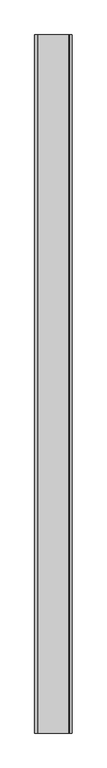
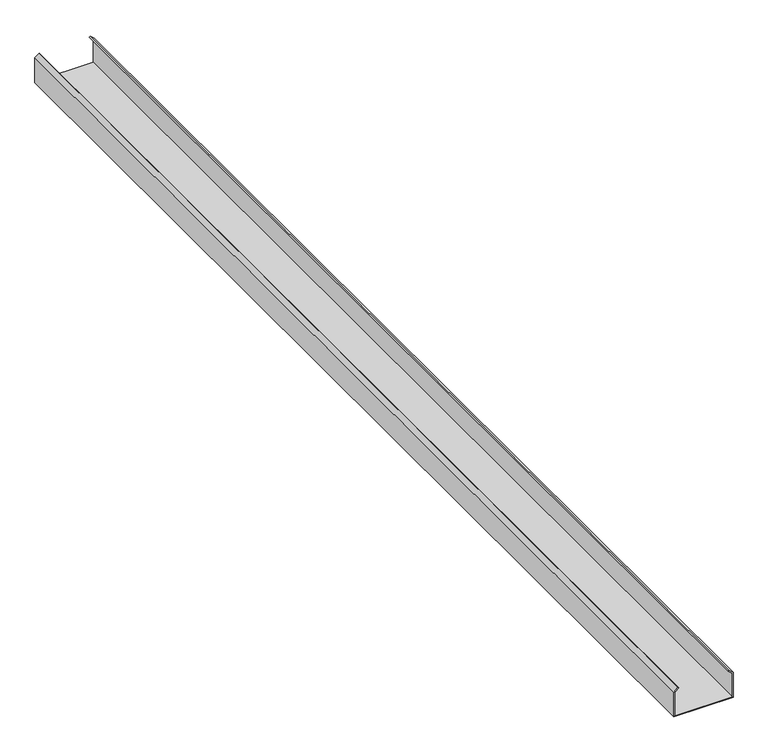
"""IFC4 building model written with IfcOpenShell, lengths in millimetres: proxy geometry, Generic Models 7:Generic Models 1:1:Generic Models 1:1 : Generic Models 7:Generic Models 1:337419:51 : Generic Models 7:Generic Models 1:1:Generic Models 1:1 : Generic Models 7:Generic Models 1:337419:306201."""

from ifc_helpers import new_model, si_unit, frame, origin, place, context, project, spatial, polyline, outline, extrude, source, transform, mapped, element, save


def generic_models_450da2eb(model_context):
    return source(origin(), model_context, "Body", "SweptSolid", [
        extrude(outline(polyline([(3617.9125, 560568.8617239), (3706.8125, 560568.8617239), (3719.057604, 560554.2685773), (3716.9294367, 560552.482833), (3705.517039, 560566.0835989), (3620.690625, 560566.0835989), (3620.690625, 560368.4398489), (3705.517039, 560368.4398489), (3716.9294367, 560382.0406149), (3719.057604, 560380.2548706), (3706.8125, 560365.6617239), (3617.9125, 560365.6617239), (3617.9125, 560568.8617239)])), frame((0.0, -546971.2913841, 0.0), z_axis=(0.0, 1.0, 0.0), x_axis=(0.0, 0.0, 1.0)), (0.0, 0.0, 1.0), 3787.775),
    ])


if __name__ == "__main__":
    model = new_model("IFC4")
    model_context = context("Model", 3, world=origin())
    ifc_project = project(units=[si_unit("LENGTHUNIT", "METRE", prefix="MILLI")], contexts=[model_context])
    site = spatial("IfcSite", under=ifc_project)
    building = spatial("IfcBuilding", under=site)
    placement = place(None, origin())
    generic_models_shape = generic_models_450da2eb(model_context)
    element("IfcBuildingElementProxy", 1, Name="Generic Models 7:Generic Models 1:1:Generic Models 1:1 : Generic Models 7:Generic Models 1:337419:51 : Generic Models 7:Generic Models 1:1:Generic Models 1:1 : Generic Models 7:Generic Models 1:337419:306201", ObjectType="Generic Models 7:Generic Models 1:1:Generic Models 1:1 : Generic Models 7:Generic Models 1:337419:51 : Generic Models 7:Generic Models 1:1:Generic Models 1:1 : Generic Models 7:Generic Models 1:337419:306201", at=placement, inside=building, context=model_context, shape_type="MappedRepresentation", body=[
        mapped(generic_models_shape, transform((0.0, 0.0, 0.0), x_axis=(1.0, 0.0, 0.0), y_axis=(0.0, 1.0, 0.0), z_axis=(0.0, 0.0, 1.0))),
    ])
    save(model, "model.ifc")

# Revit data of these elements
# Type "Generic Models 7:Generic Models 1:1:Generic Models 1:1 : Generic Models 7:Generic Models 1:337419:51 : Generic Models 7:Generic Models 1:1:Generic Models 1:1 : Generic Models 7:Generic Models 1:337419:306201"
#   NameOverride = "Generic Models 7:Generic Models 1:1:Generic Models 1:1 : Generic Models 7:Generic Models 1:337419:306201"
#   ObjectTypeOverride = "Generic Models 1:1 : Generic Models 7:Generic Models 1:337419"
#   Reference = "Generic Models 1"
#   Tag = "306201"
# Element 1 (IfcBuildingElementProxy, "Generic Models 7:Generic Models 1:1:Generic Models 1:1 : Generic Models 7:Generic Models 1:337419:51 : Generic Models 7:Generic Models 1:1:Generic Models 1:1 : Generic Models 7:Generic Models 1:337419:306201")
#   Materials on its faces: "CEE' SECTION (8.0x3.5C - SEE STRUCT. DWGS)"
# Materials
#   "CEE' SECTION (8.0x3.5C - SEE STRUCT. DWGS)": class "Unassigned", colour RGB 210 209 208, transparency 0, Keynote = "M05121300.02", Cost = 0
